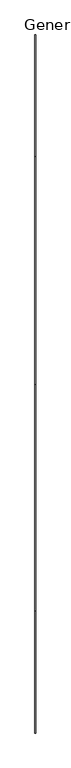
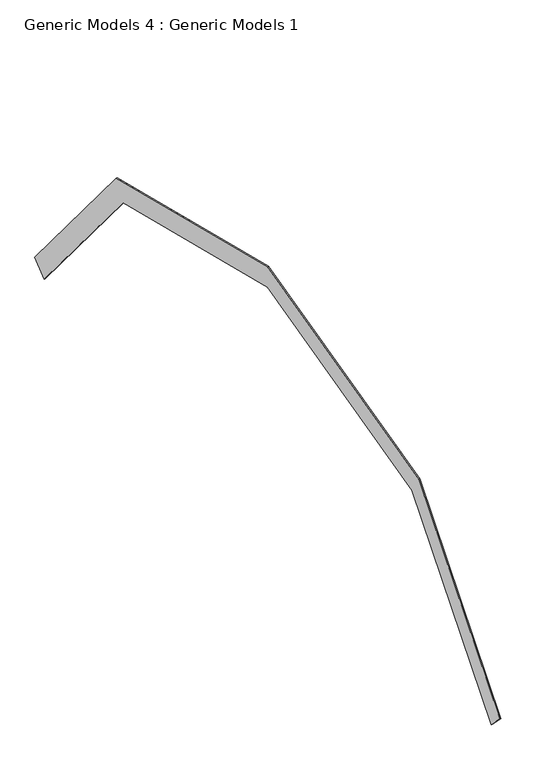
"""IFC4 building model written with IfcOpenShell, lengths in millimetres: proxy geometry, Generic Models 4 : Generic Models 1."""

import ifcopenshell
import ifcopenshell.guid

model = None  # the IFC model being written
_history = None  # IfcOwnerHistory: only IFC2X3 demands one
_inside = {}  # id of a spatial element -> (the spatial element, [elements in it])
_under = {}  # id of a project, library or spatial element -> (it, [spatial elements below it])
_declared = {}  # id of a project -> (the project, [libraries it declares])
_typed = {}  # id of a type object -> (the type object, [elements of that type])
_made_of = {}  # id of a material, layer set ... -> (it, [elements and type objects made of it])


def new_model(schema):
    """Start an empty IFC model of exactly this schema.

    Asked for "IFC4X3", IfcOpenShell would pick the latest addendum, in which some entities
    have other attributes; the version numbers below select the first issue.
    IFC2X3 requires an IfcOwnerHistory on every rooted entity: one is made here for all.
    """
    global model, _history
    if schema == "IFC4X3":
        model = ifcopenshell.file(schema_version=(4, 3, 0, 0))
    else:
        model = ifcopenshell.file(schema=schema)
    _inside.clear()
    _under.clear()
    _declared.clear()
    _typed.clear()
    _made_of.clear()
    _history = None
    if model.schema == "IFC2X3":
        org = make("IfcOrganization", Name="unknown")
        user = make(
            "IfcPersonAndOrganization",
            ThePerson=make("IfcPerson", FamilyName="unknown"),
            TheOrganization=org,
        )
        app = make(
            "IfcApplication",
            ApplicationDeveloper=org,
            Version="unknown",
            ApplicationFullName="unknown",
            ApplicationIdentifier="unknown",
        )
        _history = make(
            "IfcOwnerHistory",
            OwningUser=user,
            OwningApplication=app,
            ChangeAction="ADDED",
            CreationDate=0,
        )
    return model


def make(cls, **values):
    """One entity of the class cls with the attributes given. An attribute that is None is left unset."""
    return model.create_entity(
        cls, **{name: value for name, value in values.items() if value is not None}
    )


def rooted(cls, **values):
    """An entity with a GlobalId (a new one), such as an element, a storey or a relation."""
    return make(cls, GlobalId=ifcopenshell.guid.new(), OwnerHistory=_history, **values)


def si_unit(unit_type, name, prefix=None):
    """IfcSIUnit, for example si_unit("LENGTHUNIT", "METRE", prefix="MILLI")."""
    return make("IfcSIUnit", UnitType=unit_type, Prefix=prefix, Name=name)


def assignment(units):
    """IfcUnitAssignment: the units of a project."""
    return None if units is None else make("IfcUnitAssignment", Units=units)


def point(xyz):
    """IfcCartesianPoint."""
    return None if xyz is None else make("IfcCartesianPoint", Coordinates=xyz)


def direction(xyz):
    """IfcDirection."""
    return None if xyz is None else make("IfcDirection", DirectionRatios=xyz)


def frame(location, z_axis=None, x_axis=None):
    """IfcAxis2Placement3D, a coordinate frame: its origin and axes. An axis left out is left unset."""
    return make(
        "IfcAxis2Placement3D",
        Location=point(location),
        Axis=direction(z_axis),
        RefDirection=direction(x_axis),
    )


def origin():
    """The frame at (0, 0, 0) with its axes left unset."""
    return frame((0.0, 0.0, 0.0))


def place(relative_to, where):
    """IfcLocalPlacement: puts the frame where relative to a parent placement (None: the world)."""
    return make(
        "IfcLocalPlacement", PlacementRelTo=relative_to, RelativePlacement=where
    )


def context(
    kind, dimensions, precision=None, world=None, true_north=None, identifier=None
):
    """IfcGeometricRepresentationContext, for example the 3D "Model" context."""
    return make(
        "IfcGeometricRepresentationContext",
        ContextIdentifier=identifier,
        ContextType=kind,
        CoordinateSpaceDimension=dimensions,
        Precision=precision,
        WorldCoordinateSystem=world,
        TrueNorth=true_north,
    )


def project(units=None, contexts=None):
    """IfcProject with its units and contexts."""
    return rooted(
        "IfcProject",
        Name="project",
        RepresentationContexts=contexts,
        UnitsInContext=assignment(units),
    )


def spatial(cls, under=None, at=None, **own):
    """A site, building, storey or space (cls), placed at a placement, below another one or the project."""
    s = rooted(cls, ObjectPlacement=at, **own)
    if under is not None:
        _under.setdefault(under.id(), (under, []))[1].append(s)
    return s


def polyline(points):
    """IfcPolyline through the points."""
    return make("IfcPolyline", Points=[point(p) for p in points])


def outline(outer, holes=None, kind="AREA"):
    """IfcArbitraryClosedProfileDef: a profile drawn as a closed curve; with holes, ...WithVoids."""
    if holes is None:
        return make("IfcArbitraryClosedProfileDef", ProfileType=kind, OuterCurve=outer)
    return make(
        "IfcArbitraryProfileDefWithVoids",
        ProfileType=kind,
        OuterCurve=outer,
        InnerCurves=holes,
    )


def extrude(swept, where, along, depth):
    """IfcExtrudedAreaSolid: the profile swept, set in the frame where, extruded along a direction by depth."""
    return make(
        "IfcExtrudedAreaSolid",
        SweptArea=swept,
        Position=where,
        ExtrudedDirection=direction(along),
        Depth=depth,
    )


def shape(context_of_items, identifier, shape_type, items):
    """IfcShapeRepresentation: the items that make up one representation, for example the "Body"."""
    return make(
        "IfcShapeRepresentation",
        ContextOfItems=context_of_items,
        RepresentationIdentifier=identifier,
        RepresentationType=shape_type,
        Items=items,
    )


def source(mapping_origin, context_of_items, identifier, shape_type, items):
    """IfcRepresentationMap: a shape defined once, which mapped items show again and again."""
    return make(
        "IfcRepresentationMap",
        MappingOrigin=mapping_origin,
        MappedRepresentation=shape(context_of_items, identifier, shape_type, items),
    )


def transform(
    local_origin,
    x_axis=None,
    y_axis=None,
    z_axis=None,
    scale=None,
    scale2=None,
    scale3=None,
    uniform=True,
):
    """IfcCartesianTransformationOperator3D, or its non-uniform kind. x_axis, y_axis, z_axis: its Axis1, 2, 3."""
    if uniform:
        return make(
            "IfcCartesianTransformationOperator3D",
            Axis1=direction(x_axis),
            Axis2=direction(y_axis),
            LocalOrigin=point(local_origin),
            Scale=scale,
            Axis3=direction(z_axis),
        )
    return make(
        "IfcCartesianTransformationOperator3DnonUniform",
        Axis1=direction(x_axis),
        Axis2=direction(y_axis),
        LocalOrigin=point(local_origin),
        Scale=scale,
        Axis3=direction(z_axis),
        Scale2=scale2,
        Scale3=scale3,
    )


def mapped(mapping_source, mapping_target):
    """IfcMappedItem: shows the shape of a source again, moved by a transform."""
    return make(
        "IfcMappedItem", MappingSource=mapping_source, MappingTarget=mapping_target
    )


def made_of(thing, what):
    """Note that an element or type object is made of a material, layer set ...; save() writes the relation."""
    if what is not None:
        _made_of.setdefault(what.id(), (what, []))[1].append(thing)
    return thing


def element(
    cls,
    number,
    at=None,
    inside=None,
    cuts=None,
    type_object=None,
    material=None,
    context=None,
    identifier="Body",
    shape_type=None,
    held_by="IfcProductDefinitionShape",
    body=None,
    shapes=None,
    **own,
):
    """One element of the class cls, such as IfcWall. Its Tag is "e" and its number.

    at: its placement. inside: the storey or other place that contains it. cuts: it is an
    opening in that element (IfcRelVoidsElement). A single representation is given by context,
    identifier, shape_type and body (its items); several are given by shapes. held_by: the class
    of the entity that holds the representations. save() writes the other relations.
    """
    e = rooted(cls, Tag="e%d" % number, ObjectPlacement=at, **own)
    if body is not None:
        shapes = [shape(context, identifier, shape_type, body)]
    if shapes is not None:
        e.Representation = make(held_by, Representations=shapes)
    if inside is not None:
        _inside.setdefault(inside.id(), (inside, []))[1].append(e)
    if cuts is not None:
        rooted(
            "IfcRelVoidsElement", RelatingBuildingElement=cuts, RelatedOpeningElement=e
        )
    if type_object is not None:
        _typed.setdefault(type_object.id(), (type_object, []))[1].append(e)
    return made_of(e, material)


def aggregate(whole, parts):
    """IfcRelAggregates: a whole, such as a stair, and the parts it consists of."""
    return rooted("IfcRelAggregates", RelatingObject=whole, RelatedObjects=parts)


def save(model, path):
    """Write the relations noted so far, then the file.

    IfcRelAggregates (storeys below a building ...), IfcRelContainedInSpatialStructure (elements
    in a storey), IfcRelDefinesByType, IfcRelAssociatesMaterial and IfcRelDeclares: one each for
    every whole, place, type object, material and project.
    """
    for whole, parts in _under.values():
        aggregate(whole, parts)
    for where, things in _inside.values():
        rooted(
            "IfcRelContainedInSpatialStructure",
            RelatedElements=things,
            RelatingStructure=where,
        )
    for kind, things in _typed.values():
        rooted("IfcRelDefinesByType", RelatedObjects=things, RelatingType=kind)
    for what, things in _made_of.values():
        rooted("IfcRelAssociatesMaterial", RelatedObjects=things, RelatingMaterial=what)
    for by, libraries in _declared.values():
        rooted("IfcRelDeclares", RelatingContext=by, RelatedDefinitions=libraries)
    model.write(path)


def generic_models_4_generic_models_1_4f2df183(model_context):
    return source(origin(), model_context, "Body", "SweptSolid", [
        extrude(outline(polyline([(11606.2878096, 2984.3405795), (10019.9980933, 4887.8882391), (7109.4138362, 5615.5343034), (4198.7953154, 4887.8796732), (2604.5089175, 2974.7359957), (2431.2242181, 3148.0206952), (4062.7194377, 5105.8149588), (7110.1288453, 5867.6673107), (10157.5382529, 5105.8149588), (11793.7171223, 3142.4003155), (11606.2878096, 2984.3405795)])), frame((29947.3870052, 0.0, 0.0), z_axis=(1.0, 0.0, 0.0), x_axis=(0.0, 1.0, 0.0)), (0.0, 0.0, 1.0), 13.5023771),
    ])


if __name__ == "__main__":
    model = new_model("IFC4")
    model_context = context("Model", 3, world=origin())
    ifc_project = project(units=[si_unit("LENGTHUNIT", "METRE", prefix="MILLI")], contexts=[model_context])
    site = spatial("IfcSite", under=ifc_project)
    building = spatial("IfcBuilding", under=site)
    placement = place(None, origin())
    generic_models_4_generic_models_1_shape = generic_models_4_generic_models_1_4f2df183(model_context)
    element("IfcBuildingElementProxy", 1, Name="Generic Models 4 : Generic Models 1", ObjectType="Generic Models 4 : Generic Models 1", at=placement, inside=building, context=model_context, shape_type="MappedRepresentation", body=[
        mapped(generic_models_4_generic_models_1_shape, transform((0.0, 0.0, 0.0), x_axis=(1.0, 0.0, 0.0), y_axis=(0.0, 1.0, 0.0), z_axis=(0.0, 0.0, 1.0))),
    ])
    save(model, "model.ifc")
